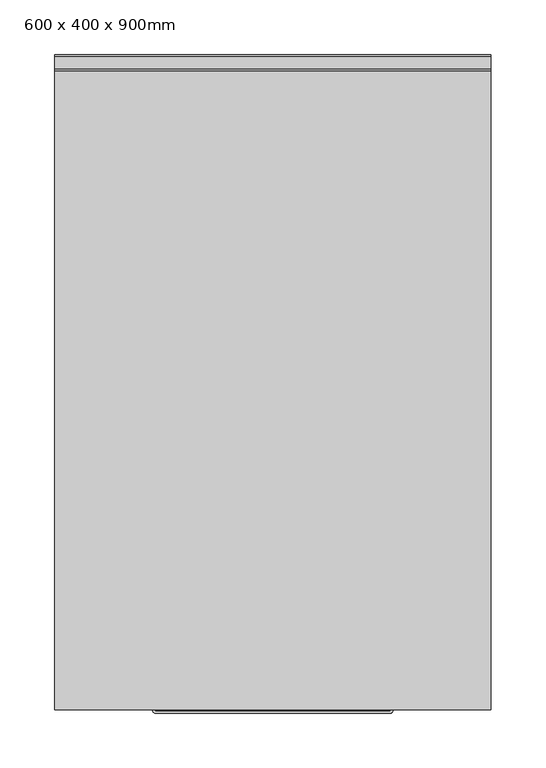
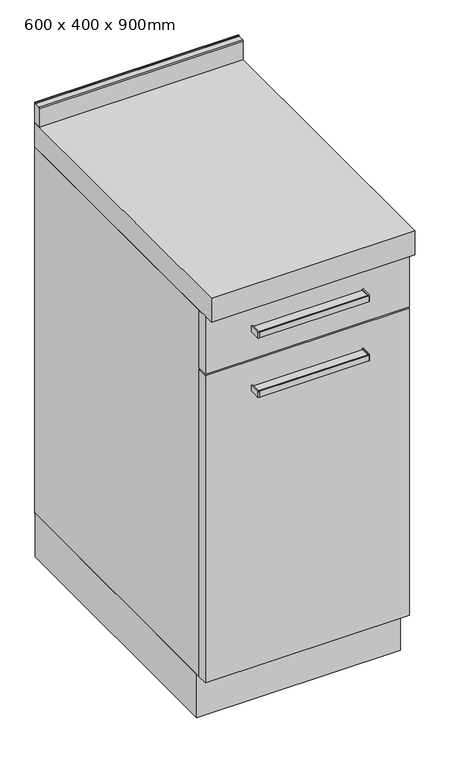
"""IFC4 building model written with IfcOpenShell, lengths in millimetres: furniture geometry, Küchenelement (1) - 1-flg - 1 Schublade : 600 x 400 x 900mm."""

from ifc_helpers import new_model, si_unit, point, frame, frame_2d, origin, origin_with_axes, place, context, project, spatial, polyline, circle_curve, trimmed, segment, composite_curve, outline, extrude, source, transform, mapped, element, save


def furniture_600_x_400_x_900mm_83104363(model_context):
    return source(origin(), model_context, "Body", "SweptSolid", [
        extrude(outline(composite_curve([segment(polyline([(-63.2996736, -580.0), (152.7003264, -580.0), (152.7003264, -600.5)]), True, "CONTINUOUS"), segment(trimmed(circle_curve(frame_2d((152.2003264, -600.5)), 0.5), [point((152.7003264, -600.5))], [point((152.2003264, -601.0))], False, "CARTESIAN"), True, "CONTINUOUS"), segment(polyline([(152.2003264, -601.0), (-62.7996736, -601.0)]), True, "CONTINUOUS"), segment(trimmed(circle_curve(frame_2d((-62.7996736, -600.5)), 0.5), [point((-62.7996736, -601.0))], [point((-63.2996736, -600.5))], False, "CARTESIAN"), True, "CONTINUOUS"), segment(polyline([(-63.2996736, -600.5), (-63.2996736, -580.0)]), True, "CONTINUOUS")], self_intersect=False)), frame((0.0, 0.0, 666.755389), z_axis=(0.0, 0.0, 1.0), x_axis=(1.0, 0.0, 0.0)), (0.0, 0.0, 1.0), 6.4890959),
        extrude(outline(composite_curve([segment(polyline([(-65.2996736, -580.0), (-63.2996736, -580.0), (-63.2996736, -600.5)]), True, "CONTINUOUS"), segment(trimmed(circle_curve(frame_2d((-62.7996736, -600.5)), 0.5), [point((-63.2996736, -600.5))], [point((-62.7996736, -601.0))], True, "CARTESIAN"), True, "CONTINUOUS"), segment(polyline([(-62.7996736, -601.0), (152.2003264, -601.0)]), True, "CONTINUOUS"), segment(trimmed(circle_curve(frame_2d((152.2003264, -600.5)), 0.5), [point((152.2003264, -601.0))], [point((152.7003264, -600.5))], True, "CARTESIAN"), True, "CONTINUOUS"), segment(polyline([(152.7003264, -600.5), (152.7003264, -580.0), (154.7003264, -580.0), (154.7003264, -600.5)]), True, "CONTINUOUS"), segment(trimmed(circle_curve(frame_2d((152.2003264, -600.5)), 2.5), [point((154.7003264, -600.5))], [point((152.2003264, -603.0))], False, "CARTESIAN"), True, "CONTINUOUS"), segment(polyline([(152.2003264, -603.0), (-62.7996736, -603.0)]), True, "CONTINUOUS"), segment(trimmed(circle_curve(frame_2d((-62.7996736, -600.5)), 2.5), [point((-62.7996736, -603.0))], [point((-65.2996736, -600.5))], False, "CARTESIAN"), True, "CONTINUOUS"), segment(polyline([(-65.2996736, -600.5), (-65.2996736, -580.0)]), True, "CONTINUOUS")], self_intersect=False)), frame((0.0, 0.0, 663.99), z_axis=(0.0, 0.0, 1.0), x_axis=(1.0, 0.0, 0.0)), (0.0, 0.0, 1.0), 12.0),
        extrude(outline(composite_curve([segment(polyline([(-63.2996736, -580.0), (152.7003264, -580.0), (152.7003264, -600.5)]), True, "CONTINUOUS"), segment(trimmed(circle_curve(frame_2d((152.2003264, -600.5)), 0.5), [point((152.7003264, -600.5))], [point((152.2003264, -601.0))], False, "CARTESIAN"), True, "CONTINUOUS"), segment(polyline([(152.2003264, -601.0), (-62.7996736, -601.0)]), True, "CONTINUOUS"), segment(trimmed(circle_curve(frame_2d((-62.7996736, -600.5)), 0.5), [point((-62.7996736, -601.0))], [point((-63.2996736, -600.5))], False, "CARTESIAN"), True, "CONTINUOUS"), segment(polyline([(-63.2996736, -600.5), (-63.2996736, -580.0)]), True, "CONTINUOUS")], self_intersect=False)), frame((0.0, 0.0, 789.785389), z_axis=(0.0, 0.0, 1.0), x_axis=(1.0, 0.0, 0.0)), (0.0, 0.0, 1.0), 6.4890959),
        extrude(outline(composite_curve([segment(polyline([(-65.2996736, -580.0), (-63.2996736, -580.0), (-63.2996736, -600.5)]), True, "CONTINUOUS"), segment(trimmed(circle_curve(frame_2d((-62.7996736, -600.5)), 0.5), [point((-63.2996736, -600.5))], [point((-62.7996736, -601.0))], True, "CARTESIAN"), True, "CONTINUOUS"), segment(polyline([(-62.7996736, -601.0), (152.2003264, -601.0)]), True, "CONTINUOUS"), segment(trimmed(circle_curve(frame_2d((152.2003264, -600.5)), 0.5), [point((152.2003264, -601.0))], [point((152.7003264, -600.5))], True, "CARTESIAN"), True, "CONTINUOUS"), segment(polyline([(152.7003264, -600.5), (152.7003264, -580.0), (154.7003264, -580.0), (154.7003264, -600.5)]), True, "CONTINUOUS"), segment(trimmed(circle_curve(frame_2d((152.2003264, -600.5)), 2.5), [point((154.7003264, -600.5))], [point((152.2003264, -603.0))], False, "CARTESIAN"), True, "CONTINUOUS"), segment(polyline([(152.2003264, -603.0), (-62.7996736, -603.0)]), True, "CONTINUOUS"), segment(trimmed(circle_curve(frame_2d((-62.7996736, -600.5)), 2.5), [point((-62.7996736, -603.0))], [point((-65.2996736, -600.5))], False, "CARTESIAN"), True, "CONTINUOUS"), segment(polyline([(-65.2996736, -600.5), (-65.2996736, -580.0)]), True, "CONTINUOUS")], self_intersect=False)), frame((0.0, 0.0, 787.02), z_axis=(0.0, 0.0, 1.0), x_axis=(1.0, 0.0, 0.0)), (0.0, 0.0, 1.0), 12.0),
        extrude(outline(polyline([(244.7003264, -580.0), (-155.2996736, -580.0), (-155.2996736, -558.0), (244.7003264, -558.0), (244.7003264, -580.0)])), frame((0.0, 0.0, 730.02), z_axis=(0.0, 0.0, 1.0), x_axis=(1.0, 0.0, 0.0)), (0.0, 0.0, 1.0), 119.98),
        extrude(outline(polyline([(244.7003264, -580.0), (-155.2996736, -580.0), (-155.2996736, -558.0), (244.7003264, -558.0), (244.7003264, -580.0)])), frame((0.0, 0.0, 90.0), z_axis=(0.0, 0.0, 1.0), x_axis=(1.0, 0.0, 0.0)), (0.0, 0.0, 1.0), 637.02),
        extrude(outline(composite_curve([segment(polyline([(0.0, 942.0034681), (0.0, 900.0), (-15.0, 900.0), (-15.0, 938.0)]), True, "CONTINUOUS"), segment(trimmed(circle_curve(frame_2d((-13.0, 938.0)), 2.0), [point((-15.0, 938.0))], [point((-13.0, 940.0))], False, "CARTESIAN"), True, "CONTINUOUS"), segment(polyline([(-13.0, 940.0), (-1.50449, 940.0), (-1.50449, 942.0034681), (0.0, 942.0034681)]), True, "CONTINUOUS")], self_intersect=False)), frame((-155.2996736, 0.0, 0.0), z_axis=(1.0, 0.0, 0.0), x_axis=(0.0, 1.0, 0.0)), (0.0, 0.0, 1.0), 400.0),
        extrude(outline(polyline([(244.7003264, -0.533703), (244.7003264, -550.533703), (-155.2996736, -550.533703), (-155.2996736, -0.533703), (244.7003264, -0.533703)])), origin_with_axes(), (0.0, 0.0, 1.0), 90.0),
        extrude(outline(polyline([(244.7003264, 0.0), (244.7003264, -600.0), (-155.2996736, -600.0), (-155.2996736, 0.0), (244.7003264, 0.0)])), frame((0.0, 0.0, 850.0), z_axis=(0.0, 0.0, 1.0), x_axis=(1.0, 0.0, 0.0)), (0.0, 0.0, 1.0), 50.0),
        extrude(outline(polyline([(244.7003264, 0.0), (244.7003264, -558.0), (222.7003264, -558.0), (222.7003264, -22.0), (-133.2996736, -22.0), (-133.2996736, -558.0), (-155.2996736, -558.0), (-155.2996736, 0.0), (244.7003264, 0.0)])), frame((0.0, 0.0, 90.0), z_axis=(0.0, 0.0, 1.0), x_axis=(1.0, 0.0, 0.0)), (0.0, 0.0, 1.0), 760.0),
    ])


if __name__ == "__main__":
    model = new_model("IFC4")
    model_context = context("Model", 3, world=origin())
    ifc_project = project(units=[si_unit("LENGTHUNIT", "METRE", prefix="MILLI")], contexts=[model_context])
    site = spatial("IfcSite", under=ifc_project)
    building = spatial("IfcBuilding", under=site)
    placement = place(None, origin())
    furniture_600_x_400_x_900mm_shape = furniture_600_x_400_x_900mm_83104363(model_context)
    element("IfcFurniture", 1, ObjectType="Küchenelement (1) - 1-flg - 1 Schublade : 600 x 400 x 900mm", at=placement, inside=building, context=model_context, shape_type="MappedRepresentation", body=[
        mapped(furniture_600_x_400_x_900mm_shape, transform((0.0, 0.0, 0.0), x_axis=(1.0, 0.0, 0.0), y_axis=(0.0, 1.0, 0.0), z_axis=(0.0, 0.0, 1.0))),
    ])
    save(model, "model.ifc")

# Revit data of these elements
# Type "Küchenelement (1) - 1-flg - 1 Schublade : 600 x 400 x 900mm"
#   Assembly Code = "C1030400"
#   Länge 3 = 0.63702 m
#   Länge 2 = 0.12303 m
#   Länge 1 = 0.10098 m
#   Depth = 0.600 m
#   Height = 0.900 m
#   Width = 0.400 m
#   Obermaterial = none
#   Material = none
#   Griffmaterial = none
# Element 1 (IfcFurniture, "Küchenelement (1) - 1-flg - 1 Schublade : 600 x 400 x 900mm")
#   Materials on its faces: "Holz - Birke"
# Materials
#   "Holz - Birke": class "Holz", colour RGB 213 164 103, transparency 0, Cost = 0
